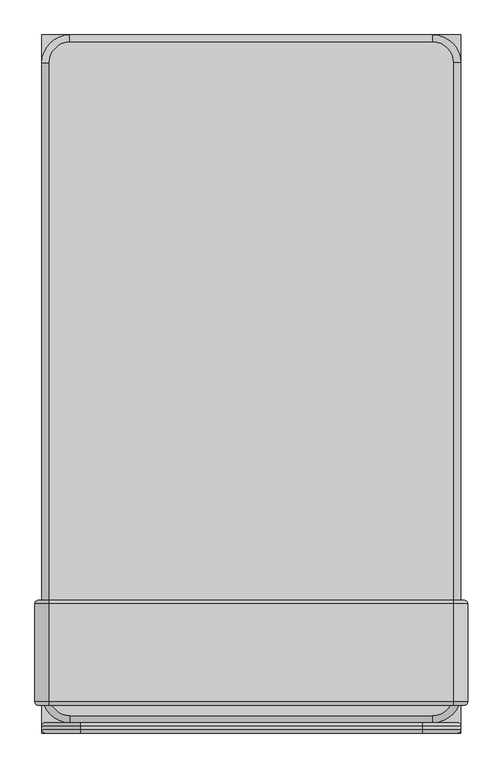
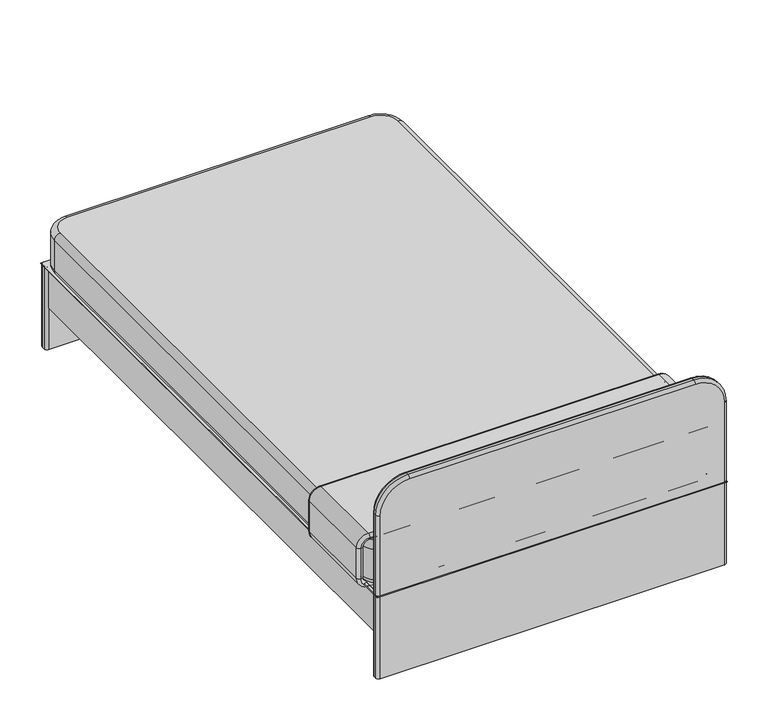
"""IFC4 building model written with IfcOpenShell, lengths in millimetres: furniture geometry, ベッド : 1200 x 2000 mm セミダブル."""

from ifc_helpers import new_model, si_unit, point, frame, frame_2d, origin, origin_with_axes, place, context, project, spatial, polyline, circle_curve, ellipse_curve, trimmed, segment, composite_curve, outline, extrude, source, transform, mapped, element, save
from ifc_brep_helpers import plane_surface, cylinder_surface, revolved_surface, advanced_brep


def furniture_c1053457(model_context):
    return source(origin(), model_context, "Body", "SolidModel", [
        advanced_brep(
        [(600.0, -960.0, 430.0), (580.0, -960.0, 450.0), (580.0, -680.0, 450.0), (600.0, -680.0, 430.0), (610.0, -970.0, 430.0), (580.0, -970.0, 460.0), (620.0, -960.0, 430.0), (580.0, -960.0, 470.0), (620.0, -680.0, 430.0), (580.0, -680.0, 470.0), (610.0, -670.0, 430.0), (580.0, -670.0, 460.0), (600.0, -680.0, 320.0), (600.0, -960.0, 320.0), (610.0, -970.0, 320.0), (620.0, -960.0, 320.0), (620.0, -680.0, 320.0), (610.0, -670.0, 320.0), (580.0, -960.0, 300.0), (580.0, -680.0, 300.0), (580.0, -970.0, 290.0), (580.0, -960.0, 280.0), (580.0, -680.0, 280.0), (580.0, -670.0, 290.0), (-580.0, -680.0, 300.0), (-580.0, -960.0, 300.0), (-580.0, -970.0, 290.0), (-580.0, -960.0, 280.0), (-580.0, -680.0, 280.0), (-580.0, -670.0, 290.0), (-600.0, -960.0, 320.0), (-600.0, -680.0, 320.0), (-610.0, -970.0, 320.0), (-620.0, -960.0, 320.0), (-620.0, -680.0, 320.0), (-610.0, -670.0, 320.0), (-600.0, -680.0, 430.0), (-600.0, -960.0, 430.0), (-610.0, -970.0, 430.0), (-620.0, -960.0, 430.0), (-620.0, -680.0, 430.0), (-610.0, -670.0, 430.0), (-580.0, -960.0, 450.0), (-580.0, -680.0, 450.0), (-580.0, -970.0, 460.0), (-580.0, -960.0, 470.0), (-580.0, -680.0, 470.0), (-580.0, -670.0, 460.0)],
        [
            (0, 1, circle_curve(frame((580.0, -960.0, 430.0), z_axis=(0.0, -1.0, 0.0), x_axis=(0.0, 0.0, 1.0)), 20.0)),
            (1, 2),
            (2, 3, circle_curve(frame((580.0, -680.0, 430.0), z_axis=(0.0, 1.0, 0.0), x_axis=(0.0, 0.0, 1.0)), 20.0)),
            (3, 0),
            (4, 5, circle_curve(frame((580.0, -970.0, 430.0), z_axis=(0.0, -1.0, 0.0), x_axis=(0.0, 0.0, 1.0)), 30.0)),
            (5, 1, circle_curve(frame((580.0, -960.0, 460.0), z_axis=(1.0, 0.0, 0.0), x_axis=(0.0, 0.0, 1.0)), 10.0)),
            (0, 4, circle_curve(frame((610.0, -960.0, 430.0), z_axis=(0.0, 0.0, 1.0), x_axis=(1.0, 0.0, 0.0)), 10.0)),
            (6, 7, circle_curve(frame((580.0, -960.0, 430.0), z_axis=(0.0, -1.0, 0.0), x_axis=(0.0, 0.0, 1.0)), 40.0)),
            (7, 5, circle_curve(frame((580.0, -960.0, 460.0), z_axis=(1.0, 0.0, 0.0), x_axis=(0.0, 0.0, 1.0)), 10.0)),
            (4, 6, circle_curve(frame((610.0, -960.0, 430.0), z_axis=(0.0, 0.0, 1.0), x_axis=(1.0, 0.0, 0.0)), 10.0)),
            (8, 9, circle_curve(frame((580.0, -680.0, 430.0), z_axis=(0.0, -1.0, 0.0), x_axis=(0.0, 0.0, 1.0)), 40.0)),
            (9, 7),
            (6, 8),
            (10, 11, circle_curve(frame((580.0, -670.0, 430.0), z_axis=(0.0, -1.0, 0.0), x_axis=(0.0, 0.0, 1.0)), 30.0)),
            (11, 9, circle_curve(frame((580.0, -680.0, 460.0), z_axis=(1.0, 0.0, 0.0), x_axis=(0.0, 0.0, 1.0)), 10.0)),
            (8, 10, circle_curve(frame((610.0, -680.0, 430.0), z_axis=(0.0, 0.0, 1.0), x_axis=(1.0, 0.0, 0.0)), 10.0)),
            (2, 11, circle_curve(frame((580.0, -680.0, 460.0), z_axis=(1.0, 0.0, 0.0), x_axis=(0.0, 0.0, 1.0)), 10.0)),
            (10, 3, circle_curve(frame((610.0, -680.0, 430.0), z_axis=(0.0, 0.0, 1.0), x_axis=(1.0, 0.0, 0.0)), 10.0)),
            (3, 12),
            (12, 13),
            (13, 0),
            (13, 14, circle_curve(frame((610.0, -960.0, 320.0), z_axis=(0.0, 0.0, 1.0), x_axis=(1.0, 0.0, 0.0)), 10.0)),
            (14, 4),
            (14, 15, circle_curve(frame((610.0, -960.0, 320.0), z_axis=(0.0, 0.0, 1.0), x_axis=(1.0, 0.0, 0.0)), 10.0)),
            (15, 6),
            (15, 16),
            (16, 8),
            (16, 17, circle_curve(frame((610.0, -680.0, 320.0), z_axis=(0.0, 0.0, 1.0), x_axis=(1.0, 0.0, 0.0)), 10.0)),
            (17, 10),
            (17, 12, circle_curve(frame((610.0, -680.0, 320.0), z_axis=(0.0, 0.0, 1.0), x_axis=(1.0, 0.0, 0.0)), 10.0)),
            (18, 13, circle_curve(frame((580.0, -960.0, 320.0), z_axis=(0.0, -1.0, 0.0), x_axis=(1.0, 0.0, 0.0)), 20.0)),
            (12, 19, circle_curve(frame((580.0, -680.0, 320.0), z_axis=(0.0, 1.0, 0.0), x_axis=(1.0, 0.0, 0.0)), 20.0)),
            (19, 18),
            (20, 14, circle_curve(frame((580.0, -970.0, 320.0), z_axis=(0.0, -1.0, 0.0), x_axis=(1.0, 0.0, 0.0)), 30.0)),
            (18, 20, circle_curve(frame((580.0, -960.0, 290.0), z_axis=(1.0, 0.0, 0.0), x_axis=(0.0, 0.0, -1.0)), 10.0)),
            (21, 15, circle_curve(frame((580.0, -960.0, 320.0), z_axis=(0.0, -1.0, 0.0), x_axis=(1.0, 0.0, 0.0)), 40.0)),
            (20, 21, circle_curve(frame((580.0, -960.0, 290.0), z_axis=(1.0, 0.0, 0.0), x_axis=(0.0, 0.0, -1.0)), 10.0)),
            (22, 16, circle_curve(frame((580.0, -680.0, 320.0), z_axis=(0.0, -1.0, 0.0), x_axis=(1.0, 0.0, 0.0)), 40.0)),
            (21, 22),
            (23, 17, circle_curve(frame((580.0, -670.0, 320.0), z_axis=(0.0, -1.0, 0.0), x_axis=(1.0, 0.0, 0.0)), 30.0)),
            (22, 23, circle_curve(frame((580.0, -680.0, 290.0), z_axis=(1.0, 0.0, 0.0), x_axis=(0.0, 0.0, -1.0)), 10.0)),
            (23, 19, circle_curve(frame((580.0, -680.0, 290.0), z_axis=(1.0, 0.0, 0.0), x_axis=(0.0, 0.0, -1.0)), 10.0)),
            (19, 24),
            (24, 25),
            (25, 18),
            (25, 26, circle_curve(frame((-580.0, -960.0, 290.0), z_axis=(1.0, 0.0, 0.0), x_axis=(0.0, 0.0, -1.0)), 10.0)),
            (26, 20),
            (26, 27, circle_curve(frame((-580.0, -960.0, 290.0), z_axis=(1.0, 0.0, 0.0), x_axis=(0.0, 0.0, -1.0)), 10.0)),
            (27, 21),
            (27, 28),
            (28, 22),
            (28, 29, circle_curve(frame((-580.0, -680.0, 290.0), z_axis=(1.0, 0.0, 0.0), x_axis=(0.0, 0.0, -1.0)), 10.0)),
            (29, 23),
            (29, 24, circle_curve(frame((-580.0, -680.0, 290.0), z_axis=(1.0, 0.0, 0.0), x_axis=(0.0, 0.0, -1.0)), 10.0)),
            (30, 25, circle_curve(frame((-580.0, -960.0, 320.0), z_axis=(0.0, -1.0, 0.0), x_axis=(0.0, 0.0, -1.0)), 20.0)),
            (24, 31, circle_curve(frame((-580.0, -680.0, 320.0), z_axis=(0.0, 1.0, 0.0), x_axis=(0.0, 0.0, -1.0)), 20.0)),
            (31, 30),
            (32, 26, circle_curve(frame((-580.0, -970.0, 320.0), z_axis=(0.0, -1.0, 0.0), x_axis=(0.0, 0.0, -1.0)), 30.0)),
            (30, 32, circle_curve(frame((-610.0, -960.0, 320.0), z_axis=(0.0, 0.0, -1.0), x_axis=(-1.0, 0.0, 0.0)), 10.0)),
            (33, 27, circle_curve(frame((-580.0, -960.0, 320.0), z_axis=(0.0, -1.0, 0.0), x_axis=(0.0, 0.0, -1.0)), 40.0)),
            (32, 33, circle_curve(frame((-610.0, -960.0, 320.0), z_axis=(0.0, 0.0, -1.0), x_axis=(-1.0, 0.0, 0.0)), 10.0)),
            (34, 28, circle_curve(frame((-580.0, -680.0, 320.0), z_axis=(0.0, -1.0, 0.0), x_axis=(0.0, 0.0, -1.0)), 40.0)),
            (33, 34),
            (35, 29, circle_curve(frame((-580.0, -670.0, 320.0), z_axis=(0.0, -1.0, 0.0), x_axis=(0.0, 0.0, -1.0)), 30.0)),
            (34, 35, circle_curve(frame((-610.0, -680.0, 320.0), z_axis=(0.0, 0.0, -1.0), x_axis=(-1.0, 0.0, 0.0)), 10.0)),
            (35, 31, circle_curve(frame((-610.0, -680.0, 320.0), z_axis=(0.0, 0.0, -1.0), x_axis=(-1.0, 0.0, 0.0)), 10.0)),
            (31, 36),
            (36, 37),
            (37, 30),
            (37, 38, circle_curve(frame((-610.0, -960.0, 430.0), z_axis=(0.0, 0.0, -1.0), x_axis=(-1.0, 0.0, 0.0)), 10.0)),
            (38, 32),
            (38, 39, circle_curve(frame((-610.0, -960.0, 430.0), z_axis=(0.0, 0.0, -1.0), x_axis=(-1.0, 0.0, 0.0)), 10.0)),
            (39, 33),
            (39, 40),
            (40, 34),
            (40, 41, circle_curve(frame((-610.0, -680.0, 430.0), z_axis=(0.0, 0.0, -1.0), x_axis=(-1.0, 0.0, 0.0)), 10.0)),
            (41, 35),
            (41, 36, circle_curve(frame((-610.0, -680.0, 430.0), z_axis=(0.0, 0.0, -1.0), x_axis=(-1.0, 0.0, 0.0)), 10.0)),
            (42, 37, circle_curve(frame((-580.0, -960.0, 430.0), z_axis=(0.0, -1.0, 0.0), x_axis=(-1.0, 0.0, 0.0)), 20.0)),
            (36, 43, circle_curve(frame((-580.0, -680.0, 430.0), z_axis=(0.0, 1.0, 0.0), x_axis=(-1.0, 0.0, 0.0)), 20.0)),
            (43, 42),
            (44, 38, circle_curve(frame((-580.0, -970.0, 430.0), z_axis=(0.0, -1.0, 0.0), x_axis=(-1.0, 0.0, 0.0)), 30.0)),
            (42, 44, circle_curve(frame((-580.0, -960.0, 460.0), z_axis=(-1.0, 0.0, 0.0), x_axis=(0.0, 0.0, 1.0)), 10.0)),
            (45, 39, circle_curve(frame((-580.0, -960.0, 430.0), z_axis=(0.0, -1.0, 0.0), x_axis=(-1.0, 0.0, 0.0)), 40.0)),
            (44, 45, circle_curve(frame((-580.0, -960.0, 460.0), z_axis=(-1.0, 0.0, 0.0), x_axis=(0.0, 0.0, 1.0)), 10.0)),
            (46, 40, circle_curve(frame((-580.0, -680.0, 430.0), z_axis=(0.0, -1.0, 0.0), x_axis=(-1.0, 0.0, 0.0)), 40.0)),
            (45, 46),
            (47, 41, circle_curve(frame((-580.0, -670.0, 430.0), z_axis=(0.0, -1.0, 0.0), x_axis=(-1.0, 0.0, 0.0)), 30.0)),
            (46, 47, circle_curve(frame((-580.0, -680.0, 460.0), z_axis=(-1.0, 0.0, 0.0), x_axis=(0.0, 0.0, 1.0)), 10.0)),
            (47, 43, circle_curve(frame((-580.0, -680.0, 460.0), z_axis=(-1.0, 0.0, 0.0), x_axis=(0.0, 0.0, 1.0)), 10.0)),
            (43, 2),
            (1, 42),
            (5, 44),
            (7, 45),
            (9, 46),
            (11, 47),
        ],
        [
            revolved_surface(polyline([(580.0, -680.0, 450.0), (580.0, -960.0, 450.0)]), (580.0, -970.0, 430.0), (0.0, 1.0, 0.0)),
            revolved_surface(trimmed(ellipse_curve(frame((580.0, -960.0, 460.0), z_axis=(-1.0, 0.0, 0.0), x_axis=(0.0, 0.0, 1.0)), 10.0, 10.0), [point((580.0, -960.0, 450.0))], [point((580.0, -970.0, 460.0))], True, "CARTESIAN"), (580.0, -970.0, 430.0), (0.0, 1.0, 0.0)),
            revolved_surface(trimmed(ellipse_curve(frame((580.0, -960.0, 460.0), z_axis=(-1.0, 0.0, 0.0), x_axis=(0.0, 0.0, 1.0)), 10.0, 10.0), [point((580.0, -970.0, 460.0))], [point((580.0, -960.0, 470.0))], True, "CARTESIAN"), (580.0, -970.0, 430.0), (0.0, 1.0, 0.0)),
            cylinder_surface(frame((580.0, -970.0, 430.0), z_axis=(0.0, 1.0, 0.0), x_axis=(0.0, 0.0, 1.0)), 40.0),
            revolved_surface(trimmed(ellipse_curve(frame((580.0, -680.0, 460.0), z_axis=(-1.0, 0.0, 0.0), x_axis=(0.0, 0.0, 1.0)), 10.0, 10.0), [point((580.0, -680.0, 470.0))], [point((580.0, -670.0, 460.0))], True, "CARTESIAN"), (580.0, -970.0, 430.0), (0.0, 1.0, 0.0)),
            revolved_surface(trimmed(ellipse_curve(frame((580.0, -680.0, 460.0), z_axis=(-1.0, 0.0, 0.0), x_axis=(0.0, 0.0, 1.0)), 10.0, 10.0), [point((580.0, -670.0, 460.0))], [point((580.0, -680.0, 450.0))], True, "CARTESIAN"), (580.0, -970.0, 430.0), (0.0, 1.0, 0.0)),
            plane_surface(frame((600.0, -680.0, 430.0), z_axis=(-1.0, 0.0, 0.0), x_axis=(0.0, 0.0, -1.0))),
            cylinder_surface(frame((610.0, -960.0, 430.0), z_axis=(0.0, 0.0, 1.0), x_axis=(1.0, 0.0, 0.0)), 10.0),
            plane_surface(frame((620.0, -960.0, 430.0), z_axis=(1.0, 0.0, 0.0), x_axis=(0.0, 0.0, -1.0))),
            cylinder_surface(frame((610.0, -680.0, 430.0), z_axis=(0.0, 0.0, 1.0), x_axis=(1.0, 0.0, 0.0)), 10.0),
            revolved_surface(polyline([(600.0, -680.0, 320.0), (600.0, -960.0, 320.0)]), (580.0, -970.0, 320.0), (0.0, 1.0, 0.0)),
            revolved_surface(trimmed(ellipse_curve(frame((610.0, -960.0, 320.0), z_axis=(0.0, 0.0, 1.0), x_axis=(1.0, 0.0, 0.0)), 10.0, 10.0), [point((600.0, -960.0, 320.0))], [point((610.0, -970.0, 320.0))], True, "CARTESIAN"), (580.0, -970.0, 320.0), (0.0, 1.0, 0.0)),
            revolved_surface(trimmed(ellipse_curve(frame((610.0, -960.0, 320.0), z_axis=(0.0, 0.0, 1.0), x_axis=(1.0, 0.0, 0.0)), 10.0, 10.0), [point((610.0, -970.0, 320.0))], [point((620.0, -960.0, 320.0))], True, "CARTESIAN"), (580.0, -970.0, 320.0), (0.0, 1.0, 0.0)),
            cylinder_surface(frame((580.0, -970.0, 320.0), z_axis=(0.0, 1.0, 0.0), x_axis=(1.0, 0.0, 0.0)), 40.0),
            revolved_surface(trimmed(ellipse_curve(frame((610.0, -680.0, 320.0), z_axis=(0.0, 0.0, 1.0), x_axis=(1.0, 0.0, 0.0)), 10.0, 10.0), [point((620.0, -680.0, 320.0))], [point((610.0, -670.0, 320.0))], True, "CARTESIAN"), (580.0, -970.0, 320.0), (0.0, 1.0, 0.0)),
            revolved_surface(trimmed(ellipse_curve(frame((610.0, -680.0, 320.0), z_axis=(0.0, 0.0, 1.0), x_axis=(1.0, 0.0, 0.0)), 10.0, 10.0), [point((610.0, -670.0, 320.0))], [point((600.0, -680.0, 320.0))], True, "CARTESIAN"), (580.0, -970.0, 320.0), (0.0, 1.0, 0.0)),
            plane_surface(frame((580.0, -680.0, 300.0), z_axis=(0.0, 0.0, 1.0), x_axis=(-1.0, 0.0, 0.0))),
            cylinder_surface(frame((580.0, -960.0, 290.0), z_axis=(1.0, 0.0, 0.0), x_axis=(0.0, 0.0, -1.0)), 10.0),
            plane_surface(frame((580.0, -960.0, 280.0), z_axis=(0.0, 0.0, -1.0), x_axis=(-1.0, 0.0, 0.0))),
            cylinder_surface(frame((580.0, -680.0, 290.0), z_axis=(1.0, 0.0, 0.0), x_axis=(0.0, 0.0, -1.0)), 10.0),
            revolved_surface(polyline([(-580.0, -680.0, 300.0), (-580.0, -960.0, 300.0)]), (-580.0, -970.0, 320.0), (0.0, 1.0, 0.0)),
            revolved_surface(trimmed(ellipse_curve(frame((-580.0, -960.0, 290.0), z_axis=(1.0, 0.0, 0.0), x_axis=(0.0, 0.0, -1.0)), 10.0, 10.0), [point((-580.0, -960.0, 300.0))], [point((-580.0, -970.0, 290.0))], True, "CARTESIAN"), (-580.0, -970.0, 320.0), (0.0, 1.0, 0.0)),
            revolved_surface(trimmed(ellipse_curve(frame((-580.0, -960.0, 290.0), z_axis=(1.0, 0.0, 0.0), x_axis=(0.0, 0.0, -1.0)), 10.0, 10.0), [point((-580.0, -970.0, 290.0))], [point((-580.0, -960.0, 280.0))], True, "CARTESIAN"), (-580.0, -970.0, 320.0), (0.0, 1.0, 0.0)),
            cylinder_surface(frame((-580.0, -970.0, 320.0), z_axis=(0.0, 1.0, 0.0), x_axis=(0.0, 0.0, -1.0)), 40.0),
            revolved_surface(trimmed(ellipse_curve(frame((-580.0, -680.0, 290.0), z_axis=(1.0, 0.0, 0.0), x_axis=(0.0, 0.0, -1.0)), 10.0, 10.0), [point((-580.0, -680.0, 280.0))], [point((-580.0, -670.0, 290.0))], True, "CARTESIAN"), (-580.0, -970.0, 320.0), (0.0, 1.0, 0.0)),
            revolved_surface(trimmed(ellipse_curve(frame((-580.0, -680.0, 290.0), z_axis=(1.0, 0.0, 0.0), x_axis=(0.0, 0.0, -1.0)), 10.0, 10.0), [point((-580.0, -670.0, 290.0))], [point((-580.0, -680.0, 300.0))], True, "CARTESIAN"), (-580.0, -970.0, 320.0), (0.0, 1.0, 0.0)),
            plane_surface(frame((-600.0, -680.0, 320.0), z_axis=(1.0, 0.0, 0.0), x_axis=(0.0, 0.0, 1.0))),
            cylinder_surface(frame((-610.0, -960.0, 320.0), z_axis=(0.0, 0.0, -1.0), x_axis=(-1.0, 0.0, 0.0)), 10.0),
            plane_surface(frame((-620.0, -960.0, 320.0), z_axis=(-1.0, 0.0, 0.0), x_axis=(0.0, 0.0, 1.0))),
            cylinder_surface(frame((-610.0, -680.0, 320.0), z_axis=(0.0, 0.0, -1.0), x_axis=(-1.0, 0.0, 0.0)), 10.0),
            revolved_surface(polyline([(-600.0, -680.0, 430.0), (-600.0, -960.0, 430.0)]), (-580.0, -970.0, 430.0), (0.0, 1.0, 0.0)),
            revolved_surface(trimmed(ellipse_curve(frame((-610.0, -960.0, 430.0), z_axis=(0.0, 0.0, -1.0), x_axis=(-1.0, 0.0, 0.0)), 10.0, 10.0), [point((-600.0, -960.0, 430.0))], [point((-610.0, -970.0, 430.0))], True, "CARTESIAN"), (-580.0, -970.0, 430.0), (0.0, 1.0, 0.0)),
            revolved_surface(trimmed(ellipse_curve(frame((-610.0, -960.0, 430.0), z_axis=(0.0, 0.0, -1.0), x_axis=(-1.0, 0.0, 0.0)), 10.0, 10.0), [point((-610.0, -970.0, 430.0))], [point((-620.0, -960.0, 430.0))], True, "CARTESIAN"), (-580.0, -970.0, 430.0), (0.0, 1.0, 0.0)),
            cylinder_surface(frame((-580.0, -970.0, 430.0), z_axis=(0.0, 1.0, 0.0), x_axis=(-1.0, 0.0, 0.0)), 40.0),
            revolved_surface(trimmed(ellipse_curve(frame((-610.0, -680.0, 430.0), z_axis=(0.0, 0.0, -1.0), x_axis=(-1.0, 0.0, 0.0)), 10.0, 10.0), [point((-620.0, -680.0, 430.0))], [point((-610.0, -670.0, 430.0))], True, "CARTESIAN"), (-580.0, -970.0, 430.0), (0.0, 1.0, 0.0)),
            revolved_surface(trimmed(ellipse_curve(frame((-610.0, -680.0, 430.0), z_axis=(0.0, 0.0, -1.0), x_axis=(-1.0, 0.0, 0.0)), 10.0, 10.0), [point((-610.0, -670.0, 430.0))], [point((-600.0, -680.0, 430.0))], True, "CARTESIAN"), (-580.0, -970.0, 430.0), (0.0, 1.0, 0.0)),
            plane_surface(frame((-580.0, -680.0, 450.0), z_axis=(0.0, 0.0, -1.0), x_axis=(1.0, 0.0, 0.0))),
            cylinder_surface(frame((-580.0, -960.0, 460.0), z_axis=(-1.0, 0.0, 0.0), x_axis=(0.0, 0.0, 1.0)), 10.0),
            plane_surface(frame((-580.0, -960.0, 470.0), z_axis=(0.0, 0.0, 1.0), x_axis=(1.0, 0.0, 0.0))),
            cylinder_surface(frame((-580.0, -680.0, 460.0), z_axis=(-1.0, 0.0, 0.0), x_axis=(0.0, 0.0, 1.0)), 10.0),
        ],
        [
            (0, [[1, 2, 3, 4]]),
            (1, [[5, 6, -1, 7]]),
            (2, [[8, 9, -5, 10]]),
            (3, [[11, 12, -8, 13]]),
            (4, [[14, 15, -11, 16]]),
            (5, [[-3, 17, -14, 18]]),
            (6, [[-4, 19, 20, 21]]),
            (7, [[-7, -21, 22, 23]]),
            (7, [[-10, -23, 24, 25]]),
            (8, [[-13, -25, 26, 27]]),
            (9, [[-16, -27, 28, 29]]),
            (9, [[-18, -29, 30, -19]]),
            (10, [[31, -20, 32, 33]]),
            (11, [[34, -22, -31, 35]]),
            (12, [[36, -24, -34, 37]]),
            (13, [[38, -26, -36, 39]]),
            (14, [[40, -28, -38, 41]]),
            (15, [[-32, -30, -40, 42]]),
            (16, [[-33, 43, 44, 45]]),
            (17, [[-35, -45, 46, 47]]),
            (17, [[-37, -47, 48, 49]]),
            (18, [[-39, -49, 50, 51]]),
            (19, [[-41, -51, 52, 53]]),
            (19, [[-42, -53, 54, -43]]),
            (20, [[55, -44, 56, 57]]),
            (21, [[58, -46, -55, 59]]),
            (22, [[60, -48, -58, 61]]),
            (23, [[62, -50, -60, 63]]),
            (24, [[64, -52, -62, 65]]),
            (25, [[-56, -54, -64, 66]]),
            (26, [[-57, 67, 68, 69]]),
            (27, [[-59, -69, 70, 71]]),
            (27, [[-61, -71, 72, 73]]),
            (28, [[-63, -73, 74, 75]]),
            (29, [[-65, -75, 76, 77]]),
            (29, [[-66, -77, 78, -67]]),
            (30, [[79, -68, 80, 81]]),
            (31, [[82, -70, -79, 83]]),
            (32, [[84, -72, -82, 85]]),
            (33, [[86, -74, -84, 87]]),
            (34, [[88, -76, -86, 89]]),
            (35, [[-80, -78, -88, 90]]),
            (36, [[-81, 91, -2, 92]]),
            (37, [[-83, -92, -6, 93]]),
            (37, [[-85, -93, -9, 94]]),
            (38, [[-87, -94, -12, 95]]),
            (39, [[-89, -95, -15, 96]]),
            (39, [[-90, -96, -17, -91]]),
        ],
    ),
        extrude(outline(polyline([(600.0, -1050.0), (-600.0, -1050.0), (-600.0, 950.0), (600.0, 950.0), (600.0, -1050.0)])), frame((0.0, 0.0, 298.0), z_axis=(0.0, 0.0, 1.0), x_axis=(1.0, 0.0, 0.0)), (0.0, 0.0, 1.0), 2.0),
        advanced_brep(
        [(600.0, -940.0, 320.0), (520.0, -1020.0, 320.0), (520.0, -1000.0, 300.0), (580.0, -940.0, 300.0), (600.0, -940.0, 430.0), (520.0, -1020.0, 430.0), (580.0, -940.0, 450.0), (520.0, -1000.0, 450.0), (580.0, 870.0, 300.0), (600.0, 870.0, 320.0), (600.0, 870.0, 430.0), (580.0, 870.0, 450.0), (520.0, 930.0, 300.0), (520.0, 950.0, 320.0), (520.0, 950.0, 430.0), (520.0, 930.0, 450.0), (-520.0, 930.0, 300.0), (-520.0, 950.0, 320.0), (-520.0, 950.0, 430.0), (-520.0, 930.0, 450.0), (-580.0, 870.0, 300.0), (-600.0, 870.0, 320.0), (-600.0, 870.0, 430.0), (-580.0, 870.0, 450.0), (-580.0, -940.0, 300.0), (-600.0, -940.0, 320.0), (-600.0, -940.0, 430.0), (-580.0, -940.0, 450.0), (-520.0, -1000.0, 300.0), (-520.0, -1020.0, 320.0), (-520.0, -1020.0, 430.0), (-520.0, -1000.0, 450.0)],
        [
            (0, 1, circle_curve(frame((520.0, -940.0, 320.0), z_axis=(0.0, 0.0, -1.0), x_axis=(0.0, -1.0, 0.0)), 80.0)),
            (1, 2, circle_curve(frame((520.0, -1000.0, 320.0), z_axis=(1.0, 0.0, 0.0), x_axis=(0.0, 1.0, 0.0)), 20.0)),
            (2, 3, circle_curve(frame((520.0, -940.0, 300.0), z_axis=(0.0, 0.0, 1.0), x_axis=(0.0, -1.0, 0.0)), 60.0)),
            (3, 0, circle_curve(frame((580.0, -940.0, 320.0), z_axis=(0.0, -1.0, 0.0), x_axis=(-1.0, 0.0, 0.0)), 20.0)),
            (0, 4),
            (4, 5, circle_curve(frame((520.0, -940.0, 430.0), z_axis=(0.0, 0.0, -1.0), x_axis=(0.0, -1.0, 0.0)), 80.0)),
            (5, 1),
            (4, 6, circle_curve(frame((580.0, -940.0, 430.0), z_axis=(0.0, -1.0, 0.0), x_axis=(-1.0, 0.0, 0.0)), 20.0)),
            (6, 7, circle_curve(frame((520.0, -940.0, 450.0), z_axis=(0.0, 0.0, -1.0), x_axis=(0.0, -1.0, 0.0)), 60.0)),
            (7, 5, circle_curve(frame((520.0, -1000.0, 430.0), z_axis=(1.0, 0.0, 0.0), x_axis=(0.0, 1.0, 0.0)), 20.0)),
            (3, 8),
            (8, 9, circle_curve(frame((580.0, 870.0, 320.0), z_axis=(0.0, -1.0, 0.0), x_axis=(-1.0, 0.0, 0.0)), 20.0)),
            (9, 0),
            (9, 10),
            (10, 4),
            (10, 11, circle_curve(frame((580.0, 870.0, 430.0), z_axis=(0.0, -1.0, 0.0), x_axis=(-1.0, 0.0, 0.0)), 20.0)),
            (11, 6),
            (8, 12, circle_curve(frame((520.0, 870.0, 300.0), z_axis=(0.0, 0.0, 1.0), x_axis=(1.0, 0.0, 0.0)), 60.0)),
            (12, 13, circle_curve(frame((520.0, 930.0, 320.0), z_axis=(1.0, 0.0, 0.0), x_axis=(0.0, -1.0, 0.0)), 20.0)),
            (13, 9, circle_curve(frame((520.0, 870.0, 320.0), z_axis=(0.0, 0.0, -1.0), x_axis=(1.0, 0.0, 0.0)), 80.0)),
            (13, 14),
            (14, 10, circle_curve(frame((520.0, 870.0, 430.0), z_axis=(0.0, 0.0, -1.0), x_axis=(1.0, 0.0, 0.0)), 80.0)),
            (14, 15, circle_curve(frame((520.0, 930.0, 430.0), z_axis=(1.0, 0.0, 0.0), x_axis=(0.0, -1.0, 0.0)), 20.0)),
            (15, 11, circle_curve(frame((520.0, 870.0, 450.0), z_axis=(0.0, 0.0, -1.0), x_axis=(1.0, 0.0, 0.0)), 60.0)),
            (12, 16),
            (16, 17, circle_curve(frame((-520.0, 930.0, 320.0), z_axis=(1.0, 0.0, 0.0), x_axis=(0.0, -1.0, 0.0)), 20.0)),
            (17, 13),
            (17, 18),
            (18, 14),
            (18, 19, circle_curve(frame((-520.0, 930.0, 430.0), z_axis=(1.0, 0.0, 0.0), x_axis=(0.0, -1.0, 0.0)), 20.0)),
            (19, 15),
            (16, 20, circle_curve(frame((-520.0, 870.0, 300.0), z_axis=(0.0, 0.0, 1.0), x_axis=(0.0, 1.0, 0.0)), 60.0)),
            (20, 21, circle_curve(frame((-580.0, 870.0, 320.0), z_axis=(0.0, 1.0, 0.0), x_axis=(1.0, 0.0, 0.0)), 20.0)),
            (21, 17, circle_curve(frame((-520.0, 870.0, 320.0), z_axis=(0.0, 0.0, -1.0), x_axis=(0.0, 1.0, 0.0)), 80.0)),
            (21, 22),
            (22, 18, circle_curve(frame((-520.0, 870.0, 430.0), z_axis=(0.0, 0.0, -1.0), x_axis=(0.0, 1.0, 0.0)), 80.0)),
            (22, 23, circle_curve(frame((-580.0, 870.0, 430.0), z_axis=(0.0, 1.0, 0.0), x_axis=(1.0, 0.0, 0.0)), 20.0)),
            (23, 19, circle_curve(frame((-520.0, 870.0, 450.0), z_axis=(0.0, 0.0, -1.0), x_axis=(0.0, 1.0, 0.0)), 60.0)),
            (20, 24),
            (24, 25, circle_curve(frame((-580.0, -940.0, 320.0), z_axis=(0.0, 1.0, 0.0), x_axis=(1.0, 0.0, 0.0)), 20.0)),
            (25, 21),
            (25, 26),
            (26, 22),
            (26, 27, circle_curve(frame((-580.0, -940.0, 430.0), z_axis=(0.0, 1.0, 0.0), x_axis=(1.0, 0.0, 0.0)), 20.0)),
            (27, 23),
            (24, 28, circle_curve(frame((-520.0, -940.0, 300.0), z_axis=(0.0, 0.0, 1.0), x_axis=(-1.0, 0.0, 0.0)), 60.0)),
            (28, 29, circle_curve(frame((-520.0, -1000.0, 320.0), z_axis=(-1.0, 0.0, 0.0), x_axis=(0.0, 1.0, 0.0)), 20.0)),
            (29, 25, circle_curve(frame((-520.0, -940.0, 320.0), z_axis=(0.0, 0.0, -1.0), x_axis=(-1.0, 0.0, 0.0)), 80.0)),
            (29, 30),
            (30, 26, circle_curve(frame((-520.0, -940.0, 430.0), z_axis=(0.0, 0.0, -1.0), x_axis=(-1.0, 0.0, 0.0)), 80.0)),
            (30, 31, circle_curve(frame((-520.0, -1000.0, 430.0), z_axis=(-1.0, 0.0, 0.0), x_axis=(0.0, 1.0, 0.0)), 20.0)),
            (31, 27, circle_curve(frame((-520.0, -940.0, 450.0), z_axis=(0.0, 0.0, -1.0), x_axis=(-1.0, 0.0, 0.0)), 60.0)),
            (31, 7),
            (2, 28),
            (1, 29),
            (5, 30),
        ],
        [
            revolved_surface(trimmed(ellipse_curve(frame((520.0, -1000.0, 320.0), z_axis=(-1.0, 0.0, 0.0), x_axis=(0.0, 1.0, 0.0)), 20.0, 20.0), [point((520.0, -1000.0, 300.0))], [point((520.0, -1020.0, 320.0))], True, "CARTESIAN"), (520.0, -940.0, 300.0), (0.0, 0.0, 1.0)),
            cylinder_surface(frame((520.0, -940.0, 300.0), z_axis=(0.0, 0.0, 1.0), x_axis=(0.0, -1.0, 0.0)), 80.0),
            revolved_surface(trimmed(ellipse_curve(frame((520.0, -1000.0, 430.0), z_axis=(-1.0, 0.0, 0.0), x_axis=(0.0, 1.0, 0.0)), 20.0, 20.0), [point((520.0, -1020.0, 430.0))], [point((520.0, -1000.0, 450.0))], True, "CARTESIAN"), (520.0, -940.0, 300.0), (0.0, 0.0, 1.0)),
            cylinder_surface(frame((580.0, -940.0, 320.0), z_axis=(0.0, -1.0, 0.0), x_axis=(-1.0, 0.0, 0.0)), 20.0),
            plane_surface(frame((600.0, -940.0, 320.0), z_axis=(1.0, 0.0, 0.0), x_axis=(0.0, 1.0, 0.0))),
            cylinder_surface(frame((580.0, -940.0, 430.0), z_axis=(0.0, -1.0, 0.0), x_axis=(-1.0, 0.0, 0.0)), 20.0),
            revolved_surface(trimmed(ellipse_curve(frame((580.0, 870.0, 320.0), z_axis=(0.0, -1.0, 0.0), x_axis=(-1.0, 0.0, 0.0)), 20.0, 20.0), [point((580.0, 870.0, 300.0))], [point((600.0, 870.0, 320.0))], True, "CARTESIAN"), (520.0, 870.0, 300.0), (0.0, 0.0, 1.0)),
            cylinder_surface(frame((520.0, 870.0, 300.0), z_axis=(0.0, 0.0, 1.0), x_axis=(1.0, 0.0, 0.0)), 80.0),
            revolved_surface(trimmed(ellipse_curve(frame((580.0, 870.0, 430.0), z_axis=(0.0, -1.0, 0.0), x_axis=(-1.0, 0.0, 0.0)), 20.0, 20.0), [point((600.0, 870.0, 430.0))], [point((580.0, 870.0, 450.0))], True, "CARTESIAN"), (520.0, 870.0, 300.0), (0.0, 0.0, 1.0)),
            cylinder_surface(frame((520.0, 930.0, 320.0), z_axis=(1.0, 0.0, 0.0), x_axis=(0.0, -1.0, 0.0)), 20.0),
            plane_surface(frame((520.0, 950.0, 320.0), z_axis=(0.0, 1.0, 0.0), x_axis=(-1.0, 0.0, 0.0))),
            cylinder_surface(frame((520.0, 930.0, 430.0), z_axis=(1.0, 0.0, 0.0), x_axis=(0.0, -1.0, 0.0)), 20.0),
            revolved_surface(trimmed(ellipse_curve(frame((-520.0, 930.0, 320.0), z_axis=(1.0, 0.0, 0.0), x_axis=(0.0, -1.0, 0.0)), 20.0, 20.0), [point((-520.0, 930.0, 300.0))], [point((-520.0, 950.0, 320.0))], True, "CARTESIAN"), (-520.0, 870.0, 300.0), (0.0, 0.0, 1.0)),
            cylinder_surface(frame((-520.0, 870.0, 300.0), z_axis=(0.0, 0.0, 1.0), x_axis=(0.0, 1.0, 0.0)), 80.0),
            revolved_surface(trimmed(ellipse_curve(frame((-520.0, 930.0, 430.0), z_axis=(1.0, 0.0, 0.0), x_axis=(0.0, -1.0, 0.0)), 20.0, 20.0), [point((-520.0, 950.0, 430.0))], [point((-520.0, 930.0, 450.0))], True, "CARTESIAN"), (-520.0, 870.0, 300.0), (0.0, 0.0, 1.0)),
            cylinder_surface(frame((-580.0, 870.0, 320.0), z_axis=(0.0, 1.0, 0.0), x_axis=(1.0, 0.0, 0.0)), 20.0),
            plane_surface(frame((-600.0, 870.0, 320.0), z_axis=(-1.0, 0.0, 0.0), x_axis=(0.0, -1.0, 0.0))),
            cylinder_surface(frame((-580.0, 870.0, 430.0), z_axis=(0.0, 1.0, 0.0), x_axis=(1.0, 0.0, 0.0)), 20.0),
            revolved_surface(trimmed(ellipse_curve(frame((-580.0, -940.0, 320.0), z_axis=(0.0, 1.0, 0.0), x_axis=(1.0, 0.0, 0.0)), 20.0, 20.0), [point((-580.0, -940.0, 300.0))], [point((-600.0, -940.0, 320.0))], True, "CARTESIAN"), (-520.0, -940.0, 300.0), (0.0, 0.0, 1.0)),
            cylinder_surface(frame((-520.0, -940.0, 300.0), z_axis=(0.0, 0.0, 1.0), x_axis=(-1.0, 0.0, 0.0)), 80.0),
            revolved_surface(trimmed(ellipse_curve(frame((-580.0, -940.0, 430.0), z_axis=(0.0, 1.0, 0.0), x_axis=(1.0, 0.0, 0.0)), 20.0, 20.0), [point((-600.0, -940.0, 430.0))], [point((-580.0, -940.0, 450.0))], True, "CARTESIAN"), (-520.0, -940.0, 300.0), (0.0, 0.0, 1.0)),
            plane_surface(frame((-520.0, -940.0, 450.0), z_axis=(0.0, 0.0, 1.0), x_axis=(-1.0, 0.0, 0.0))),
            plane_surface(frame((-520.0, -940.0, 300.0), z_axis=(0.0, 0.0, -1.0), x_axis=(-1.0, 0.0, 0.0))),
            cylinder_surface(frame((-520.0, -1000.0, 320.0), z_axis=(-1.0, 0.0, 0.0), x_axis=(0.0, 1.0, 0.0)), 20.0),
            plane_surface(frame((-520.0, -1020.0, 320.0), z_axis=(0.0, -1.0, 0.0), x_axis=(1.0, 0.0, 0.0))),
            cylinder_surface(frame((-520.0, -1000.0, 430.0), z_axis=(-1.0, 0.0, 0.0), x_axis=(0.0, 1.0, 0.0)), 20.0),
        ],
        [
            (0, [[1, 2, 3, 4]]),
            (1, [[-1, 5, 6, 7]]),
            (2, [[-6, 8, 9, 10]]),
            (3, [[-4, 11, 12, 13]]),
            (4, [[-5, -13, 14, 15]]),
            (5, [[-8, -15, 16, 17]]),
            (6, [[-12, 18, 19, 20]]),
            (7, [[-14, -20, 21, 22]]),
            (8, [[-16, -22, 23, 24]]),
            (9, [[-19, 25, 26, 27]]),
            (10, [[-21, -27, 28, 29]]),
            (11, [[-23, -29, 30, 31]]),
            (12, [[-26, 32, 33, 34]]),
            (13, [[-28, -34, 35, 36]]),
            (14, [[-30, -36, 37, 38]]),
            (15, [[-33, 39, 40, 41]]),
            (16, [[-35, -41, 42, 43]]),
            (17, [[-37, -43, 44, 45]]),
            (18, [[-40, 46, 47, 48]]),
            (19, [[-42, -48, 49, 50]]),
            (20, [[-44, -50, 51, 52]]),
            (21, [[-9, -17, -24, -31, -38, -45, -52, 53]]),
            (22, [[-3, 54, -46, -39, -32, -25, -18, -11]]),
            (23, [[-2, 55, -47, -54]]),
            (24, [[-7, 56, -49, -55]]),
            (25, [[-10, -53, -51, -56]]),
        ],
    ),
        extrude(outline(polyline([(590.0, -1020.0), (-590.0, -1020.0), (-590.0, 920.0), (590.0, 920.0), (590.0, -1020.0)])), frame((0.0, 0.0, 150.0), z_axis=(0.0, 0.0, 1.0), x_axis=(1.0, 0.0, 0.0)), (0.0, 0.0, 1.0), 150.0),
        extrude(outline(composite_curve([segment(trimmed(circle_curve(frame_2d((590.0, 940.0)), 10.0), [point((590.0, 950.0))], [point((600.0, 940.0))], False, "CARTESIAN"), True, "CONTINUOUS"), segment(polyline([(600.0, 940.0), (600.0, 930.0)]), True, "CONTINUOUS"), segment(trimmed(circle_curve(frame_2d((590.0, 930.0)), 10.0), [point((600.0, 930.0))], [point((590.0, 920.0))], False, "CARTESIAN"), True, "CONTINUOUS"), segment(polyline([(590.0, 920.0), (-590.0, 920.0)]), True, "CONTINUOUS"), segment(trimmed(circle_curve(frame_2d((-590.0, 930.0)), 10.0), [point((-590.0, 920.0))], [point((-600.0, 930.0))], False, "CARTESIAN"), True, "CONTINUOUS"), segment(polyline([(-600.0, 930.0), (-600.0, 940.0)]), True, "CONTINUOUS"), segment(trimmed(circle_curve(frame_2d((-590.0, 940.0)), 10.0), [point((-600.0, 940.0))], [point((-590.0, 950.0))], False, "CARTESIAN"), True, "CONTINUOUS"), segment(polyline([(-590.0, 950.0), (590.0, 950.0)]), True, "CONTINUOUS")], self_intersect=False)), origin_with_axes(), (0.0, 0.0, 1.0), 300.0),
        advanced_brep(
        [(-590.0, -1050.0, 0.0), (-600.0, -1040.0, 0.0), (-600.0, -1030.0, 0.0), (-590.0, -1020.0, 0.0), (590.0, -1020.0, 0.0), (600.0, -1030.0, 0.0), (600.0, -1040.0, 0.0), (590.0, -1050.0, 0.0), (590.0, -1050.0, 590.0), (490.0, -1050.0, 690.0), (-490.0, -1050.0, 690.0), (-590.0, -1050.0, 590.0), (-600.0, -1040.0, 590.0), (-600.0, -1030.0, 590.0), (-590.0, -1020.0, 590.0), (-490.0, -1020.0, 690.0), (490.0, -1020.0, 690.0), (590.0, -1020.0, 590.0), (-490.0, -1040.0, 700.0), (-490.0, -1030.0, 700.0), (490.0, -1040.0, 700.0), (490.0, -1030.0, 700.0), (600.0, -1040.0, 590.0), (600.0, -1030.0, 590.0)],
        [
            (0, 1, circle_curve(frame((-590.0, -1040.0, 0.0), z_axis=(0.0, 0.0, -1.0), x_axis=(-1.0, 0.0, 0.0)), 10.0)),
            (1, 2),
            (2, 3, circle_curve(frame((-590.0, -1030.0, 0.0), z_axis=(0.0, 0.0, -1.0), x_axis=(-1.0, 0.0, 0.0)), 10.0)),
            (3, 4),
            (4, 5, circle_curve(frame((590.0, -1030.0, 0.0), z_axis=(0.0, 0.0, -1.0), x_axis=(1.0, 0.0, 0.0)), 10.0)),
            (5, 6),
            (6, 7, circle_curve(frame((590.0, -1040.0, 0.0), z_axis=(0.0, 0.0, -1.0), x_axis=(1.0, 0.0, 0.0)), 10.0)),
            (7, 0),
            (7, 8),
            (8, 9, circle_curve(frame((490.0, -1050.0, 590.0), z_axis=(0.0, -1.0, 0.0), x_axis=(0.0, 0.0, 1.0)), 100.0)),
            (9, 10),
            (10, 11, circle_curve(frame((-490.0, -1050.0, 590.0), z_axis=(0.0, -1.0, 0.0), x_axis=(-1.0, 0.0, 0.0)), 100.0)),
            (11, 0),
            (11, 12, circle_curve(frame((-590.0, -1040.0, 590.0), z_axis=(0.0, 0.0, -1.0), x_axis=(-1.0, 0.0, 0.0)), 10.0)),
            (12, 1),
            (12, 13),
            (13, 2),
            (13, 14, circle_curve(frame((-590.0, -1030.0, 590.0), z_axis=(0.0, 0.0, -1.0), x_axis=(-1.0, 0.0, 0.0)), 10.0)),
            (14, 3),
            (14, 15, circle_curve(frame((-490.0, -1020.0, 590.0), z_axis=(0.0, 1.0, 0.0), x_axis=(-1.0, 0.0, 0.0)), 100.0)),
            (15, 16),
            (16, 17, circle_curve(frame((490.0, -1020.0, 590.0), z_axis=(0.0, 1.0, 0.0), x_axis=(0.0, 0.0, 1.0)), 100.0)),
            (17, 4),
            (10, 18, circle_curve(frame((-490.0, -1040.0, 690.0), z_axis=(-1.0, 0.0, 0.0), x_axis=(0.0, 0.0, 1.0)), 10.0)),
            (18, 12, circle_curve(frame((-490.0, -1040.0, 590.0), z_axis=(0.0, -1.0, 0.0), x_axis=(-1.0, 0.0, 0.0)), 110.0)),
            (18, 19),
            (19, 13, circle_curve(frame((-490.0, -1030.0, 590.0), z_axis=(0.0, -1.0, 0.0), x_axis=(-1.0, 0.0, 0.0)), 110.0)),
            (19, 15, circle_curve(frame((-490.0, -1030.0, 690.0), z_axis=(-1.0, 0.0, 0.0), x_axis=(0.0, 0.0, 1.0)), 10.0)),
            (9, 20, circle_curve(frame((490.0, -1040.0, 690.0), z_axis=(-1.0, 0.0, 0.0), x_axis=(0.0, 0.0, 1.0)), 10.0)),
            (20, 18),
            (20, 21),
            (21, 19),
            (21, 16, circle_curve(frame((490.0, -1030.0, 690.0), z_axis=(-1.0, 0.0, 0.0), x_axis=(0.0, 0.0, 1.0)), 10.0)),
            (8, 22, circle_curve(frame((590.0, -1040.0, 590.0), z_axis=(0.0, 0.0, 1.0), x_axis=(1.0, 0.0, 0.0)), 10.0)),
            (22, 20, circle_curve(frame((490.0, -1040.0, 590.0), z_axis=(0.0, -1.0, 0.0), x_axis=(0.0, 0.0, 1.0)), 110.0)),
            (22, 23),
            (23, 21, circle_curve(frame((490.0, -1030.0, 590.0), z_axis=(0.0, -1.0, 0.0), x_axis=(0.0, 0.0, 1.0)), 110.0)),
            (23, 17, circle_curve(frame((590.0, -1030.0, 590.0), z_axis=(0.0, 0.0, 1.0), x_axis=(1.0, 0.0, 0.0)), 10.0)),
            (6, 22),
            (5, 23),
        ],
        [
            plane_surface(frame((-540.0, -1113.2455532, 0.0), z_axis=(0.0, 0.0, -1.0), x_axis=(1.0, 0.0, 0.0))),
            plane_surface(frame((-540.0, -1050.0, 0.0), z_axis=(0.0, -1.0, 0.0), x_axis=(0.0, 0.0, 1.0))),
            cylinder_surface(frame((-590.0, -1040.0, 0.0), z_axis=(0.0, 0.0, -1.0), x_axis=(-1.0, 0.0, 0.0)), 10.0),
            plane_surface(frame((-600.0, -1040.0, 0.0), z_axis=(-1.0, 0.0, 0.0), x_axis=(0.0, 0.0, 1.0))),
            cylinder_surface(frame((-590.0, -1030.0, 0.0), z_axis=(0.0, 0.0, -1.0), x_axis=(-1.0, 0.0, 0.0)), 10.0),
            plane_surface(frame((-590.0, -1020.0, 0.0), z_axis=(0.0, 1.0, 0.0), x_axis=(0.0, 0.0, 1.0))),
            revolved_surface(trimmed(ellipse_curve(frame((-590.0, -1040.0, 590.0), z_axis=(0.0, 0.0, -1.0), x_axis=(-1.0, 0.0, 0.0)), 10.0, 10.0), [point((-590.0, -1050.0, 590.0))], [point((-600.0, -1040.0, 590.0))], True, "CARTESIAN"), (-490.0, -1050.0, 590.0), (0.0, 1.0, 0.0)),
            cylinder_surface(frame((-490.0, -1050.0, 590.0), z_axis=(0.0, 1.0, 0.0), x_axis=(-1.0, 0.0, 0.0)), 110.0),
            revolved_surface(trimmed(ellipse_curve(frame((-590.0, -1030.0, 590.0), z_axis=(0.0, 0.0, -1.0), x_axis=(-1.0, 0.0, 0.0)), 10.0, 10.0), [point((-600.0, -1030.0, 590.0))], [point((-590.0, -1020.0, 590.0))], True, "CARTESIAN"), (-490.0, -1050.0, 590.0), (0.0, 1.0, 0.0)),
            cylinder_surface(frame((-490.0, -1040.0, 690.0), z_axis=(-1.0, 0.0, 0.0), x_axis=(0.0, 0.0, 1.0)), 10.0),
            plane_surface(frame((-490.0, -1040.0, 700.0), z_axis=(0.0, 0.0, 1.0), x_axis=(1.0, 0.0, 0.0))),
            cylinder_surface(frame((-490.0, -1030.0, 690.0), z_axis=(-1.0, 0.0, 0.0), x_axis=(0.0, 0.0, 1.0)), 10.0),
            revolved_surface(trimmed(ellipse_curve(frame((490.0, -1040.0, 690.0), z_axis=(-1.0, 0.0, 0.0), x_axis=(0.0, 0.0, 1.0)), 10.0, 10.0), [point((490.0, -1050.0, 690.0))], [point((490.0, -1040.0, 700.0))], True, "CARTESIAN"), (490.0, -1050.0, 590.0), (0.0, 1.0, 0.0)),
            cylinder_surface(frame((490.0, -1050.0, 590.0), z_axis=(0.0, 1.0, 0.0), x_axis=(0.0, 0.0, 1.0)), 110.0),
            revolved_surface(trimmed(ellipse_curve(frame((490.0, -1030.0, 690.0), z_axis=(-1.0, 0.0, 0.0), x_axis=(0.0, 0.0, 1.0)), 10.0, 10.0), [point((490.0, -1030.0, 700.0))], [point((490.0, -1020.0, 690.0))], True, "CARTESIAN"), (490.0, -1050.0, 590.0), (0.0, 1.0, 0.0)),
            cylinder_surface(frame((590.0, -1040.0, 590.0), z_axis=(0.0, 0.0, 1.0), x_axis=(1.0, 0.0, 0.0)), 10.0),
            plane_surface(frame((600.0, -1040.0, 590.0), z_axis=(1.0, 0.0, 0.0), x_axis=(0.0, 0.0, -1.0))),
            cylinder_surface(frame((590.0, -1030.0, 590.0), z_axis=(0.0, 0.0, 1.0), x_axis=(1.0, 0.0, 0.0)), 10.0),
        ],
        [
            (0, [[1, 2, 3, 4, 5, 6, 7, 8]]),
            (1, [[-8, 9, 10, 11, 12, 13]]),
            (2, [[-1, -13, 14, 15]]),
            (3, [[-2, -15, 16, 17]]),
            (4, [[-3, -17, 18, 19]]),
            (5, [[-4, -19, 20, 21, 22, 23]]),
            (6, [[-12, 24, 25, -14]]),
            (7, [[-16, -25, 26, 27]]),
            (8, [[-18, -27, 28, -20]]),
            (9, [[-11, 29, 30, -24]]),
            (10, [[-26, -30, 31, 32]]),
            (11, [[-21, -28, -32, 33]]),
            (12, [[-10, 34, 35, -29]]),
            (13, [[-31, -35, 36, 37]]),
            (14, [[-22, -33, -37, 38]]),
            (15, [[-9, -7, 39, -34]]),
            (16, [[-36, -39, -6, 40]]),
            (17, [[-23, -38, -40, -5]]),
        ],
    ),
    ])


if __name__ == "__main__":
    model = new_model("IFC4")
    model_context = context("Model", 3, world=origin())
    ifc_project = project(units=[si_unit("LENGTHUNIT", "METRE", prefix="MILLI")], contexts=[model_context])
    site = spatial("IfcSite", under=ifc_project)
    building = spatial("IfcBuilding", under=site)
    placement = place(None, origin())
    furniture_shape = furniture_c1053457(model_context)
    element("IfcFurniture", 1, ObjectType="ベッド : 1200 x 2000 mm セミダブル", at=placement, inside=building, context=model_context, shape_type="MappedRepresentation", body=[
        mapped(furniture_shape, transform((0.0, 0.0, 0.0), x_axis=(1.0, 0.0, 0.0), y_axis=(0.0, 1.0, 0.0), z_axis=(0.0, 0.0, 1.0))),
    ])
    save(model, "model.ifc")

# Revit data of these elements
# Type "ベッド : 1200 x 2000 mm セミダブル"
#   Keynote = "12490.FF1"
#   幅 = 1200 mm
#   奥行き = 2000 mm
#   本体 = 木目 - ナチュラル
#   シーツ = モチアミ - 無地 - ホワイト
#   Default Elevation = 0
# Element 1 (IfcFurniture, "ベッド : 1200 x 2000 mm セミダブル")
#   Materials on its faces: "モチアミ - 無地 - ホワイト", "木目 - ナチュラル"
# Materials
#   "木目 - ナチュラル": class "木材", colour RGB 204 173 122, transparency 0, Cost = 0
#   "モチアミ - 無地 - ホワイト": class "モチアミ", colour RGB 239 232 223, transparency 0, Cost = 0
